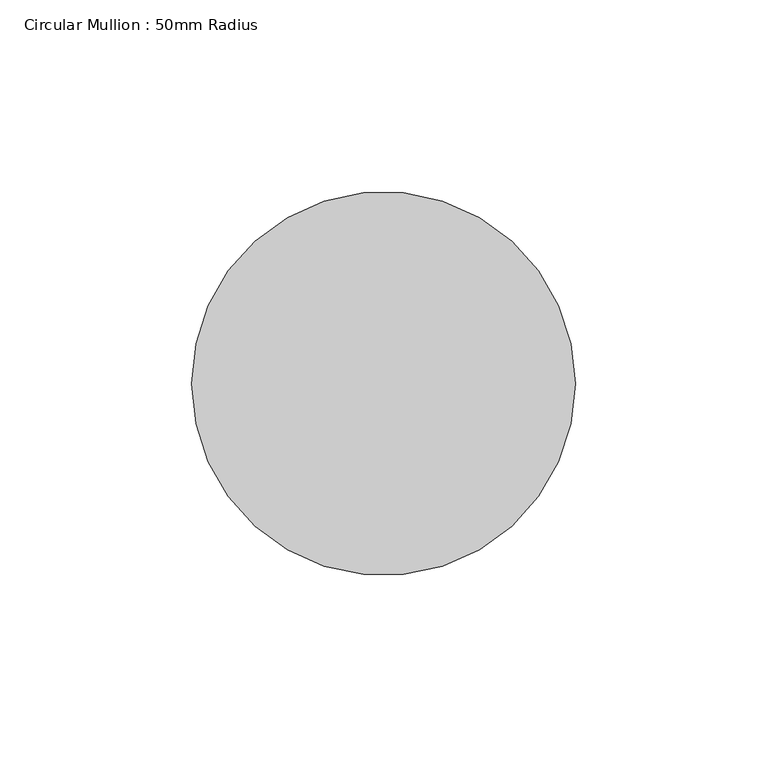
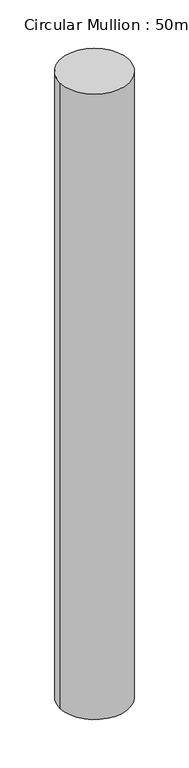
"""IFC4 building model written with IfcOpenShell, lengths in millimetres: member geometry, Circular Mullion : 50mm Radius."""

from ifc_helpers import new_model, si_unit, point, frame, origin, origin_2d, place, context, project, spatial, circle_curve, trimmed, segment, composite_curve, outline, extrude, source, transform, mapped, element, save


def circular_mullion_50mm_radius_dda96cec(model_context):
    return source(origin(), model_context, "Body", "SweptSolid", [
        extrude(outline(composite_curve([segment(trimmed(circle_curve(origin_2d(), 50.0), [point((50.0, 0.0))], [point((-50.0, 0.0))], False, "CARTESIAN"), True, "CONTINUOUS"), segment(trimmed(circle_curve(origin_2d(), 50.0), [point((-50.0, 0.0))], [point((50.0, 0.0))], False, "CARTESIAN"), True, "CONTINUOUS")], self_intersect=False)), frame((0.0, 0.0, -956.2865305), z_axis=(0.0, 0.0, 1.0), x_axis=(1.0, 0.0, 0.0)), (0.0, 0.0, 1.0), 956.2865305),
    ])


if __name__ == "__main__":
    model = new_model("IFC4")
    model_context = context("Model", 3, world=origin())
    ifc_project = project(units=[si_unit("LENGTHUNIT", "METRE", prefix="MILLI")], contexts=[model_context])
    site = spatial("IfcSite", under=ifc_project)
    building = spatial("IfcBuilding", under=site)
    placement = place(None, origin())
    circular_mullion_50mm_radius_shape = circular_mullion_50mm_radius_dda96cec(model_context)
    element("IfcMember", 1, ObjectType="Circular Mullion : 50mm Radius", at=placement, inside=building, context=model_context, shape_type="MappedRepresentation", body=[
        mapped(circular_mullion_50mm_radius_shape, transform((0.0, 0.0, 0.0), x_axis=(1.0, 0.0, 0.0), y_axis=(0.0, 1.0, 0.0), z_axis=(0.0, 0.0, 1.0))),
    ])
    save(model, "model.ifc")

# Revit data of these elements
# Type "Circular Mullion : 50mm Radius"
#   built-in parameter 1007350 = 0.164042 (stored number, unit not read)
# Element 1 (IfcMember, "Circular Mullion : 50mm Radius")
#   Materials on its faces: "Aluminium"
# Materials
#   "Aluminium": class "Metal", colour RGB 247 247 247, transparency 0, Description = "Aluminium 6061", Cost = 0
